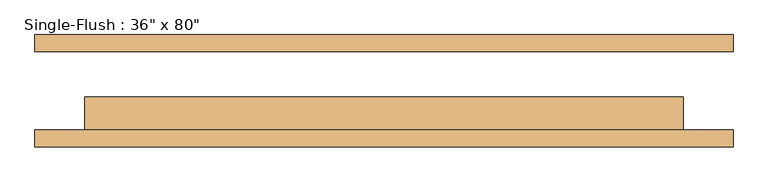
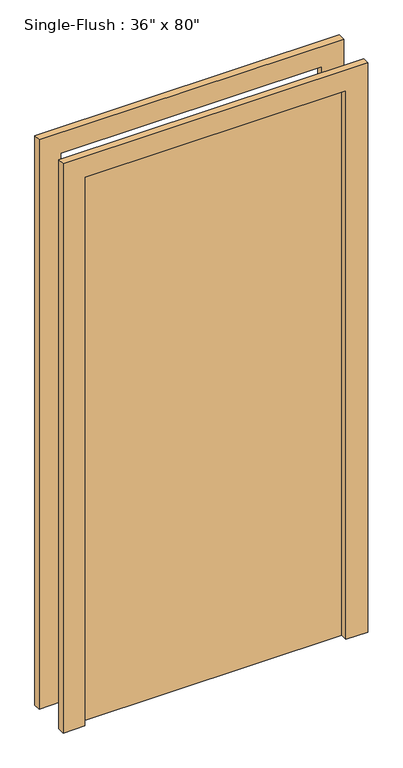
"""IFC4 building model written with IfcOpenShell, lengths in millimetres: door geometry."""

from ifc_helpers import new_model, si_unit, frame, origin, origin_with_axes, place, context, project, spatial, polyline, outline, extrude, source, transform, mapped, element, save


def door_bbe2d7fb(model_context):
    return source(origin(), model_context, "Body", "SweptSolid", [
        extrude(outline(polyline([(2108.2, -533.4), (0.0, -533.4), (0.0, -457.2), (2032.0, -457.2), (2032.0, 457.2), (0.0, 457.2), (0.0, 533.4), (2108.2, 533.4), (2108.2, -533.4)])), frame((0.0, -85.725, 0.0), z_axis=(0.0, 1.0, 0.0), x_axis=(0.0, 0.0, 1.0)), (0.0, 0.0, 1.0), 25.4),
        extrude(outline(polyline([(2108.2, 533.4), (2108.2, -533.4), (0.0, -533.4), (0.0, -457.2), (2032.0, -457.2), (2032.0, 457.2), (0.0, 457.2), (0.0, 533.4), (2108.2, 533.4)])), frame((0.0, 60.325, 0.0), z_axis=(0.0, 1.0, 0.0), x_axis=(0.0, 0.0, 1.0)), (0.0, 0.0, 1.0), 25.4),
        extrude(outline(polyline([(457.2, -9.525), (457.2, -60.325), (-457.2, -60.325), (-457.2, -9.525), (457.2, -9.525)])), origin_with_axes(), (0.0, 0.0, 1.0), 2032.0),
    ])


if __name__ == "__main__":
    model = new_model("IFC4")
    model_context = context("Model", 3, world=origin())
    ifc_project = project(units=[si_unit("LENGTHUNIT", "METRE", prefix="MILLI")], contexts=[model_context])
    site = spatial("IfcSite", under=ifc_project)
    building = spatial("IfcBuilding", under=site)
    placement = place(None, origin())
    door_shape = door_bbe2d7fb(model_context)
    element("IfcDoor", 1, ObjectType="Single-Flush : 36\" x 80\"", at=placement, inside=building, context=model_context, shape_type="MappedRepresentation", body=[
        mapped(door_shape, transform((0.0, 0.0, 0.0), x_axis=(1.0, 0.0, 0.0), y_axis=(0.0, 1.0, 0.0), z_axis=(0.0, 0.0, 1.0))),
    ])
    save(model, "model.ifc")

# Revit data of these elements
# Type "Single-Flush : 36\" x 80\""
#   Type Mark = "6"
#   Assembly Code = "C1020"
#   Thickness = 0' - 2"
#   Height = 6' - 8"
#   Trim Projection Ext = 0' - 1"
#   Trim Projection Int = 0' - 1"
#   Trim Width = 0' - 3"
#   Width = 3' - 0"
#   Door Material = drywall
#   Frame Material = drywall
#   Function = (empty or 0)
#   Wall Closure = (empty or 0)
# Element 1 (IfcDoor, "Single-Flush : 36\" x 80\"")
#   Materials on its faces: "drywall"
# Materials
#   "drywall": class "Generic", colour RGB 255 255 255, transparency 0, Description = "Gypsum Wall Board", Cost = 0
